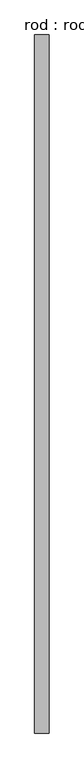
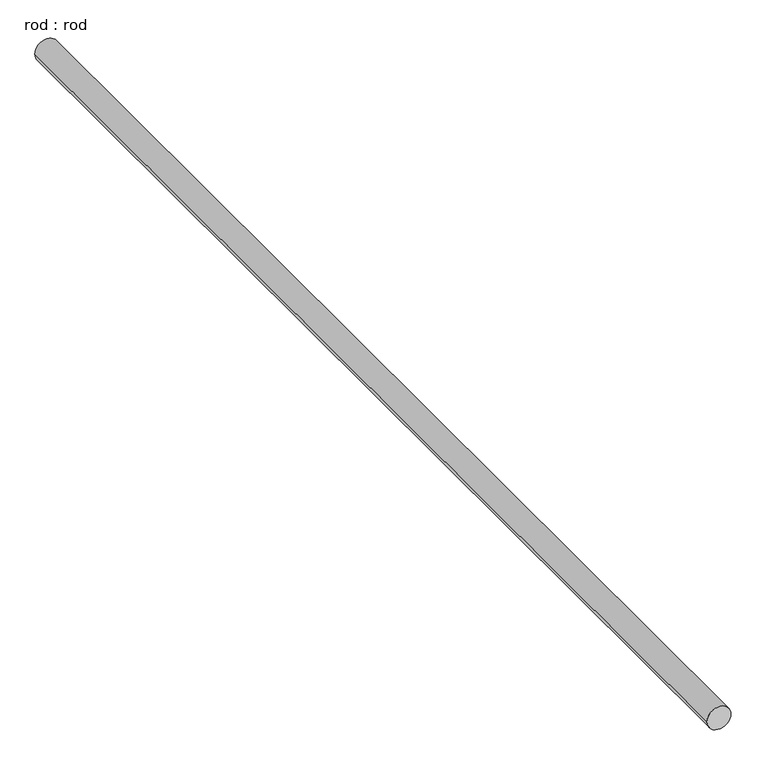
"""IFC4 building model written with IfcOpenShell, lengths in millimetres: proxy geometry, rod : rod."""

from ifc_helpers import new_model, si_unit, point, frame, frame_2d, origin, place, context, project, spatial, circle_curve, trimmed, segment, composite_curve, outline, extrude, source, transform, mapped, element, save


def rod_rod_94a62696(model_context):
    return source(origin(), model_context, "Body", "SweptSolid", [
        extrude(outline(composite_curve([segment(trimmed(circle_curve(frame_2d((0.0108462, 0.0)), 200.0), [point((0.0108462, 200.0))], [point((0.0108462, -200.0))], False, "CARTESIAN"), True, "CONTINUOUS"), segment(trimmed(circle_curve(frame_2d((0.0108462, 0.0)), 200.0), [point((0.0108462, -200.0))], [point((0.0108462, 200.0))], False, "CARTESIAN"), True, "CONTINUOUS")], self_intersect=False)), frame((0.0, -5657.2713847, 0.0), z_axis=(0.0, 1.0, 0.0), x_axis=(0.0, 0.0, 1.0)), (0.0, 0.0, 1.0), 19500.0),
    ])


if __name__ == "__main__":
    model = new_model("IFC4")
    model_context = context("Model", 3, world=origin())
    ifc_project = project(units=[si_unit("LENGTHUNIT", "METRE", prefix="MILLI")], contexts=[model_context])
    site = spatial("IfcSite", under=ifc_project)
    building = spatial("IfcBuilding", under=site)
    placement = place(None, origin())
    rod_rod_shape = rod_rod_94a62696(model_context)
    element("IfcBuildingElementProxy", 1, Name="rod : rod", ObjectType="rod : rod", at=placement, inside=building, context=model_context, shape_type="MappedRepresentation", body=[
        mapped(rod_rod_shape, transform((0.0, 0.0, 0.0), x_axis=(1.0, 0.0, 0.0), y_axis=(0.0, 1.0, 0.0), z_axis=(0.0, 0.0, 1.0))),
    ])
    save(model, "model.ifc")

# Revit data of these elements
# Type "rod : rod"
#   Default Elevation = 0
